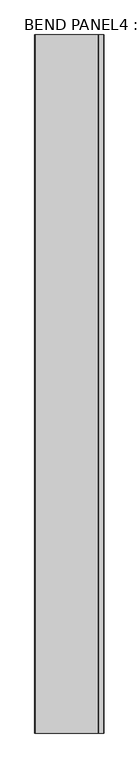
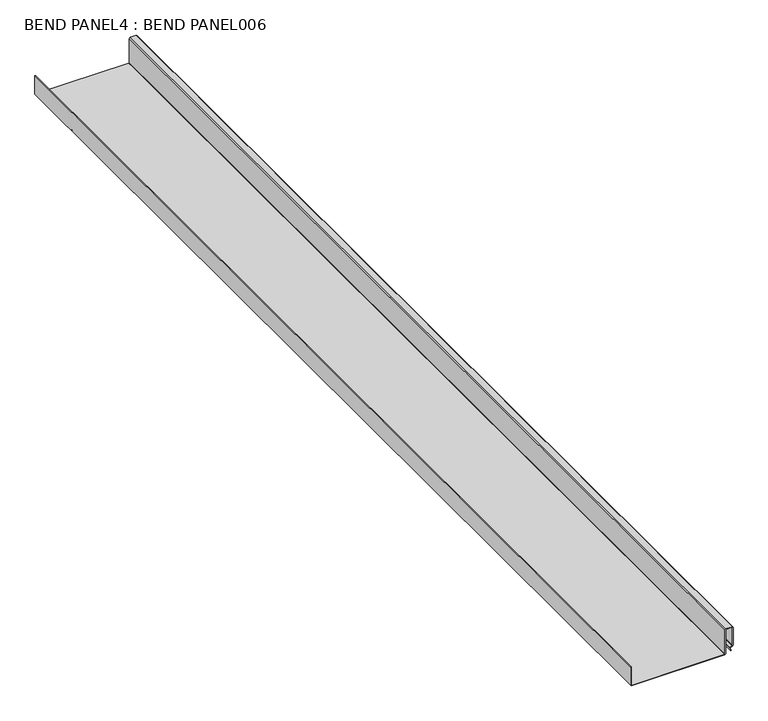
"""IFC4 building model written with IfcOpenShell, lengths in millimetres: proxy geometry, BEND PANEL4 : BEND PANEL006."""

from ifc_helpers import new_model, si_unit, frame, origin, place, context, project, spatial, polyline, outline, extrude, source, transform, mapped, element, save


def bend_panel4_bend_panel006_57896d7d(model_context):
    return source(origin(), model_context, "Body", "SweptSolid", [
        extrude(outline(polyline([(44154.5056709, 5566.2069601), (44159.1273864, 5564.0518188), (44160.0585891, 5564.3907489), (44161.9880579, 5568.5284574), (44163.8383079, 5569.6999083), (44200.0982886, 5569.6999083), (44202.1939085, 5567.6042884), (44202.1939085, 5555.919751), (44200.0982886, 5553.824131), (44151.1211561, 5553.824131), (44150.4204401, 5553.1234151), (44150.4204401, 5372.9667912), (44151.1224658, 5372.2647656), (44187.8898128, 5372.2647656), (44187.8898128, 5371.0741405), (44150.6292927, 5371.0741405), (44149.2298151, 5372.4736182), (44149.2298151, 5553.6165881), (44150.6279831, 5555.014756), (44199.6051155, 5555.014756), (44201.0032835, 5556.412924), (44201.0032835, 5567.1111154), (44199.6051156, 5568.5092833), (44164.1835313, 5568.5092833), (44162.919698, 5567.7091111), (44160.9292349, 5563.4406013), (44159.0711731, 5562.7643222), (44154.0024911, 5565.1278874), (44154.5056709, 5566.2069601)])), frame((0.0, -1052.891, 0.0), z_axis=(0.0, 1.0, 0.0), x_axis=(0.0, 0.0, 1.0)), (0.0, 0.0, 1.0), 1999.85),
    ])


if __name__ == "__main__":
    model = new_model("IFC4")
    model_context = context("Model", 3, world=origin())
    ifc_project = project(units=[si_unit("LENGTHUNIT", "METRE", prefix="MILLI")], contexts=[model_context])
    site = spatial("IfcSite", under=ifc_project)
    building = spatial("IfcBuilding", under=site)
    placement = place(None, origin())
    bend_panel4_bend_panel006_shape = bend_panel4_bend_panel006_57896d7d(model_context)
    element("IfcBuildingElementProxy", 1, Name="BEND PANEL4 : BEND PANEL006", ObjectType="BEND PANEL4 : BEND PANEL006", at=placement, inside=building, context=model_context, shape_type="MappedRepresentation", body=[
        mapped(bend_panel4_bend_panel006_shape, transform((0.0, 0.0, 0.0), x_axis=(1.0, 0.0, 0.0), y_axis=(0.0, 1.0, 0.0), z_axis=(0.0, 0.0, 1.0))),
    ])
    save(model, "model.ifc")

# Revit data of these elements
# Type "BEND PANEL4 : BEND PANEL006"
#   NameOverride = "BEND PANEL006"
# Element 1 (IfcBuildingElementProxy, "BEND PANEL4 : BEND PANEL006")
#   Materials on its faces: "STANDING SEAM METAL ROOF FOLLOW MANU. RECOMMENDED EDGE/TRANSITION DETAILS"
# Materials
#   "STANDING SEAM METAL ROOF FOLLOW MANU. RECOMMENDED EDGE/TRANSITION DETAILS": class "Unassigned", colour RGB 128 128 128, transparency 0, Cost = 0
